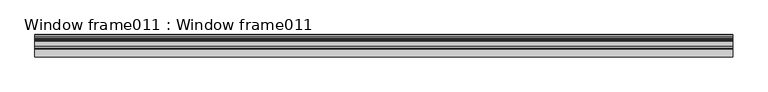
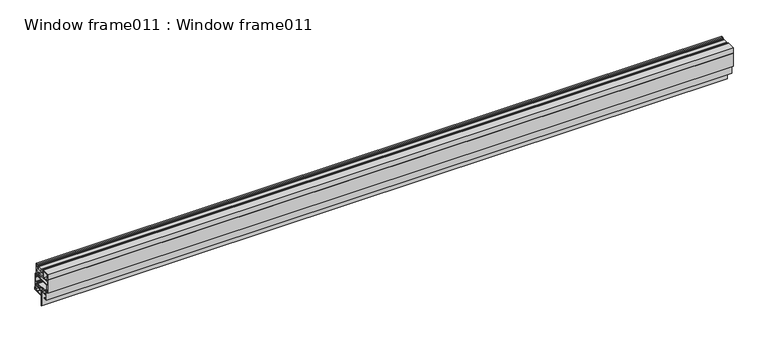
"""IFC4 building model written with IfcOpenShell, lengths in millimetres: proxy geometry, Window frame011 : Window frame011."""

from ifc_helpers import new_model, si_unit, frame, origin, place, context, project, spatial, polyline, outline, extrude, source, transform, mapped, element, save


def window_frame011_window_frame011_5eb14756(model_context):
    return source(origin(), model_context, "Body", "SweptSolid", [
        extrude(outline(polyline([(-4639.5309365, 38491.7529282), (-4640.7050488, 38491.7529282), (-4641.3675759, 38494.3431458), (-4641.3675759, 38496.2045087), (-4640.7319367, 38499.0664849), (-4639.3785718, 38499.0664849), (-4638.9548305, 38496.607592), (-4636.7286164, 38496.607592), (-4636.7286164, 38494.194592), (-4638.9555243, 38494.194592), (-4639.5309365, 38491.7529282)])), frame((12383.0178845, 0.0, 0.0), z_axis=(1.0, 0.0, 0.0), x_axis=(0.0, 1.0, 0.0)), (0.0, 0.0, 1.0), 2000.0),
        extrude(outline(polyline([(-4669.1560964, 38498.5305421), (-4667.9819841, 38498.5305421), (-4667.319457, 38495.9403245), (-4667.319457, 38494.0789616), (-4667.9550962, 38491.2169854), (-4669.3084611, 38491.2169854), (-4669.7322024, 38493.6758783), (-4671.9584164, 38493.6758783), (-4671.9584164, 38496.0888783), (-4669.7315086, 38496.0888783), (-4669.1560964, 38498.5305421)])), frame((12383.0178845, 0.0, 0.0), z_axis=(1.0, 0.0, 0.0), x_axis=(0.0, 1.0, 0.0)), (0.0, 0.0, 1.0), 2000.0),
        extrude(outline(polyline([(-4686.0427164, 38440.9919782), (-4686.8742969, 38440.9919782), (-4686.8742969, 38443.9402247), (-4690.1702164, 38443.9402247), (-4690.1702164, 38445.1340247), (-4686.8742969, 38445.1340247), (-4686.8742969, 38448.5093603), (-4686.0427164, 38448.5093603), (-4686.0427164, 38440.9919782)])), frame((12383.0178845, 0.0, 0.0), z_axis=(1.0, 0.0, 0.0), x_axis=(0.0, 1.0, 0.0)), (0.0, 0.0, 1.0), 2000.0),
        extrude(outline(polyline([(-4634.8744164, 38464.541409), (-4634.042836, 38464.541409), (-4634.042836, 38461.5931625), (-4630.7469164, 38461.5931625), (-4630.7469164, 38460.3993625), (-4634.042836, 38460.3993625), (-4634.042836, 38457.0240269), (-4634.8744164, 38457.0240269), (-4634.8744164, 38464.541409)])), frame((12383.0178845, 0.0, 0.0), z_axis=(1.0, 0.0, 0.0), x_axis=(0.0, 1.0, 0.0)), (0.0, 0.0, 1.0), 2000.0),
        extrude(outline(polyline([(-4639.3829164, 38415.5175625), (-4639.3829164, 38417.5495625), (-4630.9247164, 38417.5495625), (-4630.9247164, 38428.7001625), (-4634.7347164, 38428.7001625), (-4634.7347164, 38432.7968735), (-4633.3117065, 38432.7968735), (-4633.3117065, 38430.7768719), (-4630.9247164, 38430.7768719), (-4630.9247164, 38440.2825625), (-4633.3123168, 38440.2825625), (-4633.3123168, 38438.4776199), (-4634.7347164, 38438.4776199), (-4634.7347164, 38440.2825625), (-4636.3613739, 38440.2825625), (-4636.3613739, 38442.3145625), (-4633.2869164, 38442.3145625), (-4633.2869164, 38459.1287739), (-4632.0258979, 38459.1287739), (-4632.0258979, 38458.2403625), (-4630.7469164, 38458.2403625), (-4630.7469164, 38463.3203625), (-4632.0169164, 38463.3203625), (-4632.0169164, 38462.3291676), (-4633.2869164, 38462.3291676), (-4633.2869164, 38464.5903625), (-4628.8927164, 38464.5903625), (-4628.8927164, 38415.5175625), (-4639.3829164, 38415.5175625)])), frame((12383.0178845, 0.0, 0.0), z_axis=(1.0, 0.0, 0.0), x_axis=(0.0, 1.0, 0.0)), (0.0, 0.0, 1.0), 2000.0),
        extrude(outline(polyline([(-4649.4159164, 38478.4841625), (-4651.5876164, 38478.4841625), (-4651.5876164, 38479.8557625), (-4648.0150337, 38479.8557625), (-4648.0150337, 38476.6807625), (-4646.287204, 38476.6807625), (-4646.287204, 38474.6487661), (-4650.8764164, 38474.6487661), (-4650.8764164, 38465.0983625), (-4648.3200073, 38465.0983625), (-4648.3200073, 38466.3435796), (-4647.0664164, 38466.3435796), (-4647.0664164, 38463.0663625), (-4687.6302164, 38463.0663625), (-4687.6302164, 38446.2202428), (-4688.9233832, 38446.2202428), (-4688.9233832, 38447.1271184), (-4690.1702164, 38447.1271184), (-4690.1702164, 38442.0633061), (-4688.9241561, 38442.0633061), (-4688.9241561, 38443.0603154), (-4687.6302164, 38443.0603154), (-4687.6302164, 38440.7905625), (-4692.0244164, 38440.7905625), (-4692.0244164, 38481.5067625), (-4688.5748922, 38481.5067625), (-4689.9924164, 38478.7119161), (-4689.9924164, 38476.6807625), (-4649.4159164, 38476.6807625), (-4649.4159164, 38478.4841625)]), holes=[polyline([(-4689.4844164, 38466.2413625), (-4652.9084164, 38466.2413625), (-4652.9084164, 38473.5057625), (-4689.4844164, 38473.5057625), (-4689.4844164, 38466.2413625)])]), frame((12383.0178845, 0.0, 0.0), z_axis=(1.0, 0.0, 0.0), x_axis=(0.0, 1.0, 0.0)), (0.0, 0.0, 1.0), 2000.0),
        extrude(outline(polyline([(-4642.727462, 38486.2565625), (-4640.962162, 38484.730671), (-4640.962162, 38479.9593991), (-4639.2686164, 38479.9593991), (-4639.2686164, 38476.6807625), (-4646.0866776, 38476.6807625), (-4646.0866776, 38480.3781447), (-4653.0000564, 38480.3781447), (-4653.0000564, 38478.5294536), (-4667.0435164, 38478.5095625), (-4667.0435164, 38486.2565625), (-4642.727462, 38486.2565625)])), frame((12383.0178845, 0.0, 0.0), z_axis=(1.0, 0.0, 0.0), x_axis=(0.0, 1.0, 0.0)), (0.0, 0.0, 1.0), 2000.0),
        extrude(outline(polyline([(12383.0178845, -4660.7189164), (12383.0178845, -4647.9427164), (14383.0178845, -4647.9427164), (14383.0178845, -4660.7189164), (12383.0178845, -4660.7189164)])), frame((0.0, 0.0, 38486.2565625), z_axis=(0.0, 0.0, 1.0), x_axis=(1.0, 0.0, 0.0)), (0.0, 0.0, 1.0), 9.525),
        extrude(outline(polyline([(-4636.9064164, 38463.0663625), (-4640.6951408, 38463.0663625), (-4640.6951408, 38466.3571904), (-4639.4738693, 38466.3571904), (-4639.4738693, 38465.0983625), (-4636.9064164, 38465.0983625), (-4636.9064164, 38474.6487661), (-4641.5038161, 38474.6487661), (-4641.5038161, 38476.6807625), (-4639.2686164, 38476.6807625), (-4639.2686164, 38493.4699376), (-4638.0088043, 38493.4699376), (-4638.0088043, 38492.6065625), (-4636.7286164, 38492.6065625), (-4636.7286164, 38497.6865625), (-4638.0264587, 38497.6865625), (-4638.0264587, 38496.7026189), (-4639.2686164, 38496.7026189), (-4639.2686164, 38498.9565625), (-4634.8744164, 38498.9565625), (-4634.8744164, 38458.2403625), (-4636.9064164, 38458.2403625), (-4636.9064164, 38463.0663625)])), frame((12383.0178845, 0.0, 0.0), z_axis=(1.0, 0.0, 0.0), x_axis=(0.0, 1.0, 0.0)), (0.0, 0.0, 1.0), 2000.0),
        extrude(outline(polyline([(-4642.3510612, 38430.7321625), (-4642.3510612, 38432.7968735), (-4641.0847164, 38432.7968735), (-4641.0847164, 38428.7001625), (-4660.6427173, 38428.7001622), (-4660.6427164, 38415.4976298), (-4660.6427164, 38385.1700298), (-4662.2175164, 38385.1700298), (-4662.2175164, 38428.7001625), (-4684.0107164, 38428.7001625), (-4684.0107164, 38417.5495625), (-4675.5525164, 38417.5495625), (-4675.5525164, 38415.5175625), (-4686.0427164, 38415.5175625), (-4686.0427164, 38447.1405625), (-4682.6339998, 38447.1405625), (-4684.0107164, 38444.5748048), (-4684.0107164, 38442.3145625), (-4643.3560584, 38442.3145625), (-4643.3560584, 38444.1179625), (-4646.293591, 38444.1179625), (-4646.293591, 38445.4895625), (-4642.0574073, 38445.4895625), (-4642.0574073, 38442.3145625), (-4640.3055043, 38442.3145625), (-4640.3055043, 38440.2825625), (-4644.8947164, 38440.2825625), (-4644.8947164, 38430.7321625), (-4642.3510612, 38430.7321625)]), holes=[polyline([(-4653.8842334, 38439.1395625), (-4653.8842334, 38440.2825625), (-4662.2140522, 38440.2825625), (-4662.2140522, 38439.1395625), (-4666.1105117, 38439.1395625), (-4666.1105117, 38440.2825625), (-4670.5952491, 38440.2825625), (-4670.5952491, 38439.1395625), (-4679.4756188, 38439.1395625), (-4679.4756188, 38440.2825625), (-4683.5027164, 38440.2825625), (-4683.5027164, 38430.7321625), (-4679.5213594, 38430.7321625), (-4679.5213594, 38431.8751625), (-4675.6009273, 38431.8751625), (-4675.6009273, 38430.7321625), (-4666.0374507, 38430.7321625), (-4666.0374507, 38431.8751625), (-4660.3350067, 38431.8751625), (-4660.3350067, 38430.7321625), (-4650.5636291, 38430.7321625), (-4650.5636291, 38431.8751625), (-4646.9267164, 38431.8751625), (-4646.9267164, 38439.1395625), (-4653.8842334, 38439.1395625)])]), frame((12383.0178845, 0.0, 0.0), z_axis=(1.0, 0.0, 0.0), x_axis=(0.0, 1.0, 0.0)), (0.0, 0.0, 1.0), 2000.0),
        extrude(outline(polyline([(-4692.0244164, 38498.9565625), (-4669.4060287, 38498.9565625), (-4669.4060287, 38496.7478001), (-4670.6448459, 38496.7478001), (-4670.6448459, 38497.6769078), (-4671.9584164, 38497.6769078), (-4671.9584164, 38492.6065625), (-4670.6122465, 38492.6065625), (-4670.6122465, 38493.5040562), (-4669.438631, 38493.5040562), (-4669.438631, 38491.3204396), (-4671.9584164, 38491.3204396), (-4671.9584164, 38478.5095625), (-4649.4159164, 38478.4841625), (-4649.4159164, 38477.1125625), (-4673.3554164, 38477.1125625), (-4673.3554164, 38497.5595625), (-4690.6274164, 38497.5595625), (-4690.6274164, 38482.9037625), (-4687.201703, 38482.9037625), (-4687.201703, 38477.8169759), (-4688.0078306, 38477.8169759), (-4689.5028424, 38479.2632191), (-4688.5096075, 38481.5067625), (-4692.0244164, 38481.5067625), (-4692.0244164, 38498.9565625)])), frame((12383.0178845, 0.0, 0.0), z_axis=(1.0, 0.0, 0.0), x_axis=(0.0, 1.0, 0.0)), (0.0, 0.0, 1.0), 2000.0),
        extrude(outline(polyline([(-4660.6427164, 38383.7675625), (-4660.6427164, 38415.5175625), (-4628.8927164, 38415.5175625), (-4628.8927164, 38421.8675625), (-4627.8767164, 38421.8675625), (-4627.8767164, 38414.5015625), (-4659.6267164, 38414.5015625), (-4659.6267164, 38383.7675625), (-4660.6427164, 38383.7675625)])), frame((12383.0178845, 0.0, 0.0), z_axis=(1.0, 0.0, 0.0), x_axis=(0.0, 1.0, 0.0)), (0.0, 0.0, 1.0), 2000.0),
    ])


if __name__ == "__main__":
    model = new_model("IFC4")
    model_context = context("Model", 3, world=origin())
    ifc_project = project(units=[si_unit("LENGTHUNIT", "METRE", prefix="MILLI")], contexts=[model_context])
    site = spatial("IfcSite", under=ifc_project)
    building = spatial("IfcBuilding", under=site)
    placement = place(None, origin())
    window_frame011_window_frame011_shape = window_frame011_window_frame011_5eb14756(model_context)
    element("IfcBuildingElementProxy", 1, Name="Window frame011 : Window frame011", ObjectType="Window frame011 : Window frame011", at=placement, inside=building, context=model_context, shape_type="MappedRepresentation", body=[
        mapped(window_frame011_window_frame011_shape, transform((0.0, 0.0, 0.0), x_axis=(1.0, 0.0, 0.0), y_axis=(0.0, 1.0, 0.0), z_axis=(0.0, 0.0, 1.0))),
    ])
    save(model, "model.ifc")

# Revit data of these elements
# Type "Window frame011 : Window frame011"
#   NameOverride = "Window frame011"
# Element 1 (IfcBuildingElementProxy, "Window frame011 : Window frame011")
#   Materials on its faces: "FLEETWOOD SERIES 250-T-01 CASEMENT WINDOW FRAME"
# Materials
#   "FLEETWOOD SERIES 250-T-01 CASEMENT WINDOW FRAME": class "Unassigned", colour RGB 128 128 128, transparency 0
